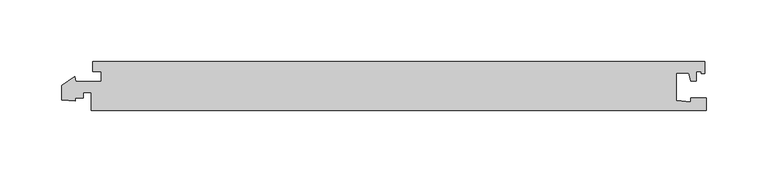
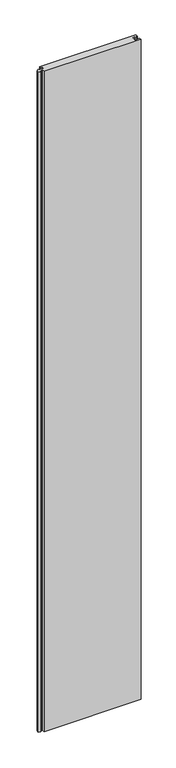
"""IFC4 building model written with IfcOpenShell, lengths in millimetres: proxy geometry, Generic Models 5:Generic Models 5:321804:Generic Models 5:321804 : Generic Models 5:Generic Models 5:321804:2 : Generic Models 5:Generic Models 5:321804:Generic Models 5:321804 : Generic Models 5:Generic Models 5:321804:300761."""

from ifc_helpers import new_model, si_unit, frame, origin, place, context, project, spatial, polyline, outline, extrude, source, transform, mapped, element, save


def generic_models_cbcfaa50(model_context):
    return source(origin(), model_context, "Body", "SweptSolid", [
        extrude(outline(polyline([(592220.2261126, -579052.1037319), (592209.8677824, -579052.1037319), (592209.8677824, -579074.5995222), (592221.8677824, -579075.6493861), (592221.8677824, -579072.4037319), (592234.6177824, -579072.4037319), (592234.6177824, -579082.6037319), (591734.6177824, -579082.6037319), (591734.6177824, -579068.1037319), (591727.9927824, -579068.1037319), (591727.9927824, -579072.4037319), (591721.3677824, -579072.4037319), (591721.3677824, -579075.1037319), (591710.3677824, -579074.1413566), (591710.3677824, -579062.2832156), (591721.0492843, -579055.1758504), (591722.101757, -579059.1037319), (591742.8177824, -579059.1037319), (591742.8177824, -579051.1037319), (591735.8677824, -579051.1037319), (591735.8677824, -579042.6037319), (592233.3677824, -579042.6037319), (592233.3677824, -579052.6037319), (592230.3677824, -579052.6037319), (592230.3677824, -579051.1037319), (592226.4177824, -579051.1037319), (592226.4177824, -579058.6037319), (592221.9677824, -579058.6037319), (592220.2261126, -579052.1037319)])), frame((0.0, 0.0, 68.8810568), z_axis=(0.0, 0.0, 1.0), x_axis=(1.0, 0.0, 0.0)), (0.0, 0.0, 1.0), 3595.9825169),
    ])


if __name__ == "__main__":
    model = new_model("IFC4")
    model_context = context("Model", 3, world=origin())
    ifc_project = project(units=[si_unit("LENGTHUNIT", "METRE", prefix="MILLI")], contexts=[model_context])
    site = spatial("IfcSite", under=ifc_project)
    building = spatial("IfcBuilding", under=site)
    placement = place(None, origin())
    generic_models_shape = generic_models_cbcfaa50(model_context)
    element("IfcBuildingElementProxy", 1, Name="Generic Models 5:Generic Models 5:321804:Generic Models 5:321804 : Generic Models 5:Generic Models 5:321804:2 : Generic Models 5:Generic Models 5:321804:Generic Models 5:321804 : Generic Models 5:Generic Models 5:321804:300761", ObjectType="Generic Models 5:Generic Models 5:321804:Generic Models 5:321804 : Generic Models 5:Generic Models 5:321804:2 : Generic Models 5:Generic Models 5:321804:Generic Models 5:321804 : Generic Models 5:Generic Models 5:321804:300761", at=placement, inside=building, context=model_context, shape_type="MappedRepresentation", body=[
        mapped(generic_models_shape, transform((0.0, 0.0, 0.0), x_axis=(1.0, 0.0, 0.0), y_axis=(0.0, 1.0, 0.0), z_axis=(0.0, 0.0, 1.0))),
    ])
    save(model, "model.ifc")

# Revit data of these elements
# Type "Generic Models 5:Generic Models 5:321804:Generic Models 5:321804 : Generic Models 5:Generic Models 5:321804:2 : Generic Models 5:Generic Models 5:321804:Generic Models 5:321804 : Generic Models 5:Generic Models 5:321804:300761"
#   NameOverride = "Generic Models 5:Generic Models 5:321804:Generic Models 5:321804 : Generic Models 5:Generic Models 5:321804:300761"
#   ObjectTypeOverride = "Generic Models 5:321804 : Generic Models 5:Generic Models 5:321804"
#   Reference = "Generic Models 5"
#   Tag = "300761"
# Element 1 (IfcBuildingElementProxy, "Generic Models 5:Generic Models 5:321804:Generic Models 5:321804 : Generic Models 5:Generic Models 5:321804:2 : Generic Models 5:Generic Models 5:321804:Generic Models 5:321804 : Generic Models 5:Generic Models 5:321804:300761")
#   Materials on its faces: "POLYCARBONATE PANEL - ARCOPLUS 547"
# Materials
#   "POLYCARBONATE PANEL - ARCOPLUS 547": class "Unassigned", colour RGB 202 225 249, transparency 0.45, Cost = 0
